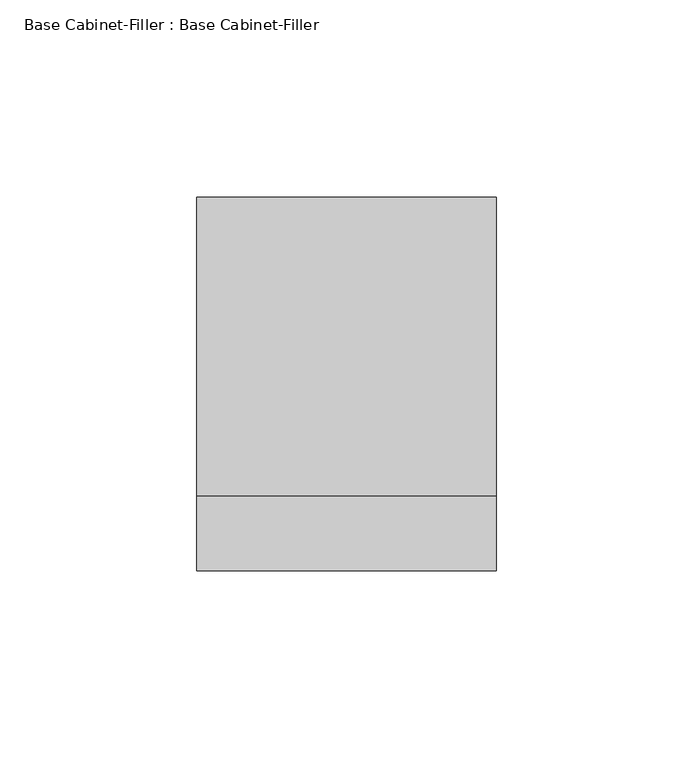
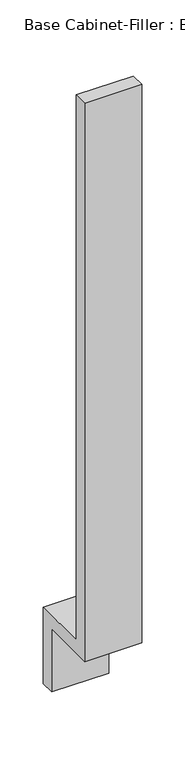
"""IFC4 building model written with IfcOpenShell, lengths in millimetres: furniture geometry, Base Cabinet-Filler : Base Cabinet-Filler."""

import ifcopenshell
import ifcopenshell.guid

model = None  # the IFC model being written
_history = None  # IfcOwnerHistory: only IFC2X3 demands one
_inside = {}  # id of a spatial element -> (the spatial element, [elements in it])
_under = {}  # id of a project, library or spatial element -> (it, [spatial elements below it])
_declared = {}  # id of a project -> (the project, [libraries it declares])
_typed = {}  # id of a type object -> (the type object, [elements of that type])
_made_of = {}  # id of a material, layer set ... -> (it, [elements and type objects made of it])


def new_model(schema):
    """Start an empty IFC model of exactly this schema.

    Asked for "IFC4X3", IfcOpenShell would pick the latest addendum, in which some entities
    have other attributes; the version numbers below select the first issue.
    IFC2X3 requires an IfcOwnerHistory on every rooted entity: one is made here for all.
    """
    global model, _history
    if schema == "IFC4X3":
        model = ifcopenshell.file(schema_version=(4, 3, 0, 0))
    else:
        model = ifcopenshell.file(schema=schema)
    _inside.clear()
    _under.clear()
    _declared.clear()
    _typed.clear()
    _made_of.clear()
    _history = None
    if model.schema == "IFC2X3":
        org = make("IfcOrganization", Name="unknown")
        user = make(
            "IfcPersonAndOrganization",
            ThePerson=make("IfcPerson", FamilyName="unknown"),
            TheOrganization=org,
        )
        app = make(
            "IfcApplication",
            ApplicationDeveloper=org,
            Version="unknown",
            ApplicationFullName="unknown",
            ApplicationIdentifier="unknown",
        )
        _history = make(
            "IfcOwnerHistory",
            OwningUser=user,
            OwningApplication=app,
            ChangeAction="ADDED",
            CreationDate=0,
        )
    return model


def make(cls, **values):
    """One entity of the class cls with the attributes given. An attribute that is None is left unset."""
    return model.create_entity(
        cls, **{name: value for name, value in values.items() if value is not None}
    )


def rooted(cls, **values):
    """An entity with a GlobalId (a new one), such as an element, a storey or a relation."""
    return make(cls, GlobalId=ifcopenshell.guid.new(), OwnerHistory=_history, **values)


def si_unit(unit_type, name, prefix=None):
    """IfcSIUnit, for example si_unit("LENGTHUNIT", "METRE", prefix="MILLI")."""
    return make("IfcSIUnit", UnitType=unit_type, Prefix=prefix, Name=name)


def assignment(units):
    """IfcUnitAssignment: the units of a project."""
    return None if units is None else make("IfcUnitAssignment", Units=units)


def point(xyz):
    """IfcCartesianPoint."""
    return None if xyz is None else make("IfcCartesianPoint", Coordinates=xyz)


def direction(xyz):
    """IfcDirection."""
    return None if xyz is None else make("IfcDirection", DirectionRatios=xyz)


def frame(location, z_axis=None, x_axis=None):
    """IfcAxis2Placement3D, a coordinate frame: its origin and axes. An axis left out is left unset."""
    return make(
        "IfcAxis2Placement3D",
        Location=point(location),
        Axis=direction(z_axis),
        RefDirection=direction(x_axis),
    )


def origin():
    """The frame at (0, 0, 0) with its axes left unset."""
    return frame((0.0, 0.0, 0.0))


def place(relative_to, where):
    """IfcLocalPlacement: puts the frame where relative to a parent placement (None: the world)."""
    return make(
        "IfcLocalPlacement", PlacementRelTo=relative_to, RelativePlacement=where
    )


def context(
    kind, dimensions, precision=None, world=None, true_north=None, identifier=None
):
    """IfcGeometricRepresentationContext, for example the 3D "Model" context."""
    return make(
        "IfcGeometricRepresentationContext",
        ContextIdentifier=identifier,
        ContextType=kind,
        CoordinateSpaceDimension=dimensions,
        Precision=precision,
        WorldCoordinateSystem=world,
        TrueNorth=true_north,
    )


def project(units=None, contexts=None):
    """IfcProject with its units and contexts."""
    return rooted(
        "IfcProject",
        Name="project",
        RepresentationContexts=contexts,
        UnitsInContext=assignment(units),
    )


def spatial(cls, under=None, at=None, **own):
    """A site, building, storey or space (cls), placed at a placement, below another one or the project."""
    s = rooted(cls, ObjectPlacement=at, **own)
    if under is not None:
        _under.setdefault(under.id(), (under, []))[1].append(s)
    return s


def polyline(points):
    """IfcPolyline through the points."""
    return make("IfcPolyline", Points=[point(p) for p in points])


def outline(outer, holes=None, kind="AREA"):
    """IfcArbitraryClosedProfileDef: a profile drawn as a closed curve; with holes, ...WithVoids."""
    if holes is None:
        return make("IfcArbitraryClosedProfileDef", ProfileType=kind, OuterCurve=outer)
    return make(
        "IfcArbitraryProfileDefWithVoids",
        ProfileType=kind,
        OuterCurve=outer,
        InnerCurves=holes,
    )


def extrude(swept, where, along, depth):
    """IfcExtrudedAreaSolid: the profile swept, set in the frame where, extruded along a direction by depth."""
    return make(
        "IfcExtrudedAreaSolid",
        SweptArea=swept,
        Position=where,
        ExtrudedDirection=direction(along),
        Depth=depth,
    )


def shape(context_of_items, identifier, shape_type, items):
    """IfcShapeRepresentation: the items that make up one representation, for example the "Body"."""
    return make(
        "IfcShapeRepresentation",
        ContextOfItems=context_of_items,
        RepresentationIdentifier=identifier,
        RepresentationType=shape_type,
        Items=items,
    )


def source(mapping_origin, context_of_items, identifier, shape_type, items):
    """IfcRepresentationMap: a shape defined once, which mapped items show again and again."""
    return make(
        "IfcRepresentationMap",
        MappingOrigin=mapping_origin,
        MappedRepresentation=shape(context_of_items, identifier, shape_type, items),
    )


def transform(
    local_origin,
    x_axis=None,
    y_axis=None,
    z_axis=None,
    scale=None,
    scale2=None,
    scale3=None,
    uniform=True,
):
    """IfcCartesianTransformationOperator3D, or its non-uniform kind. x_axis, y_axis, z_axis: its Axis1, 2, 3."""
    if uniform:
        return make(
            "IfcCartesianTransformationOperator3D",
            Axis1=direction(x_axis),
            Axis2=direction(y_axis),
            LocalOrigin=point(local_origin),
            Scale=scale,
            Axis3=direction(z_axis),
        )
    return make(
        "IfcCartesianTransformationOperator3DnonUniform",
        Axis1=direction(x_axis),
        Axis2=direction(y_axis),
        LocalOrigin=point(local_origin),
        Scale=scale,
        Axis3=direction(z_axis),
        Scale2=scale2,
        Scale3=scale3,
    )


def mapped(mapping_source, mapping_target):
    """IfcMappedItem: shows the shape of a source again, moved by a transform."""
    return make(
        "IfcMappedItem", MappingSource=mapping_source, MappingTarget=mapping_target
    )


def made_of(thing, what):
    """Note that an element or type object is made of a material, layer set ...; save() writes the relation."""
    if what is not None:
        _made_of.setdefault(what.id(), (what, []))[1].append(thing)
    return thing


def element(
    cls,
    number,
    at=None,
    inside=None,
    cuts=None,
    type_object=None,
    material=None,
    context=None,
    identifier="Body",
    shape_type=None,
    held_by="IfcProductDefinitionShape",
    body=None,
    shapes=None,
    **own,
):
    """One element of the class cls, such as IfcWall. Its Tag is "e" and its number.

    at: its placement. inside: the storey or other place that contains it. cuts: it is an
    opening in that element (IfcRelVoidsElement). A single representation is given by context,
    identifier, shape_type and body (its items); several are given by shapes. held_by: the class
    of the entity that holds the representations. save() writes the other relations.
    """
    e = rooted(cls, Tag="e%d" % number, ObjectPlacement=at, **own)
    if body is not None:
        shapes = [shape(context, identifier, shape_type, body)]
    if shapes is not None:
        e.Representation = make(held_by, Representations=shapes)
    if inside is not None:
        _inside.setdefault(inside.id(), (inside, []))[1].append(e)
    if cuts is not None:
        rooted(
            "IfcRelVoidsElement", RelatingBuildingElement=cuts, RelatedOpeningElement=e
        )
    if type_object is not None:
        _typed.setdefault(type_object.id(), (type_object, []))[1].append(e)
    return made_of(e, material)


def aggregate(whole, parts):
    """IfcRelAggregates: a whole, such as a stair, and the parts it consists of."""
    return rooted("IfcRelAggregates", RelatingObject=whole, RelatedObjects=parts)


def save(model, path):
    """Write the relations noted so far, then the file.

    IfcRelAggregates (storeys below a building ...), IfcRelContainedInSpatialStructure (elements
    in a storey), IfcRelDefinesByType, IfcRelAssociatesMaterial and IfcRelDeclares: one each for
    every whole, place, type object, material and project.
    """
    for whole, parts in _under.values():
        aggregate(whole, parts)
    for where, things in _inside.values():
        rooted(
            "IfcRelContainedInSpatialStructure",
            RelatedElements=things,
            RelatingStructure=where,
        )
    for kind, things in _typed.values():
        rooted("IfcRelDefinesByType", RelatedObjects=things, RelatingType=kind)
    for what, things in _made_of.values():
        rooted("IfcRelAssociatesMaterial", RelatedObjects=things, RelatingMaterial=what)
    for by, libraries in _declared.values():
        rooted("IfcRelDeclares", RelatingContext=by, RelatedDefinitions=libraries)
    model.write(path)


def base_cabinet_filler_base_cabinet_filler_baeeb1f6(model_context):
    return source(origin(), model_context, "Body", "SweptSolid", [
        extrude(outline(polyline([(-609.6, 88.9), (-609.6, 876.3), (-590.55, 876.3), (-590.55, 107.95), (-514.35, 107.95), (-514.35, 0.0), (-533.4, 0.0), (-533.4, 88.9), (-609.6, 88.9)])), frame((-19.3622951, 0.0, 0.0), z_axis=(1.0, 0.0, 0.0), x_axis=(0.0, 1.0, 0.0)), (0.0, 0.0, 1.0), 76.2),
    ])


if __name__ == "__main__":
    model = new_model("IFC4")
    model_context = context("Model", 3, world=origin())
    ifc_project = project(units=[si_unit("LENGTHUNIT", "METRE", prefix="MILLI")], contexts=[model_context])
    site = spatial("IfcSite", under=ifc_project)
    building = spatial("IfcBuilding", under=site)
    placement = place(None, origin())
    base_cabinet_filler_base_cabinet_filler_shape = base_cabinet_filler_base_cabinet_filler_baeeb1f6(model_context)
    element("IfcFurniture", 1, ObjectType="Base Cabinet-Filler : Base Cabinet-Filler", at=placement, inside=building, context=model_context, shape_type="MappedRepresentation", body=[
        mapped(base_cabinet_filler_base_cabinet_filler_shape, transform((0.0, 0.0, 0.0), x_axis=(1.0, 0.0, 0.0), y_axis=(0.0, 1.0, 0.0), z_axis=(0.0, 0.0, 1.0))),
    ])
    save(model, "model.ifc")

# Revit data of these elements
# Type "Base Cabinet-Filler : Base Cabinet-Filler"
#   COBie.Type.CreatedBy = "doug.wood@us.ibm.com"
#   COBie.Type.CreatedOn = "2016-04-14T02:07:23"
#   COBie.Type.Name = "Casework_Base Cabinet-Filler_Base Cabinet-Filler"
#   COBie.Type.Category = "23-40 35 17 47 11 : Kitchen Casework"
#   COBie.Type.Description = "Base Cabinet-Filler_Base Cabinet-Filler"
#   COBie.Type.Manufacturer = ""
#   COBie.Type.ModelNumber = ""
#   Assembly Code = "C1030410"
#   COBie.Type.ReplacementCost = 0
#   Depth = 2' - 0"
#   Height = 2' - 10 1/2"
#   Toe Depth = 0' - 3"
#   Toe Height = 0' - 3 1/2"
#   Width [instance default] = 0' - 3"
#   COBie.Type = no
#   Cabinet Material = none
# Element 1 (IfcFurniture, "Base Cabinet-Filler : Base Cabinet-Filler")
#   Materials on its faces: "Cabinets"
# Materials
#   "Cabinets": class "Miscellaneous", colour RGB 249 249 249, transparency 0
